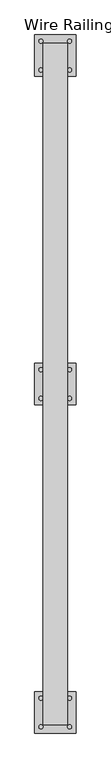
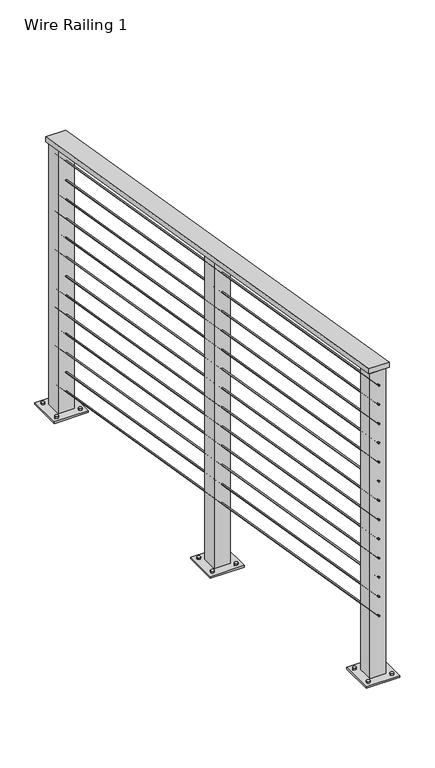
"""IFC4 building model written with IfcOpenShell, lengths in millimetres: railing geometry, Wire Railing 1."""

from ifc_helpers import new_model, si_unit, point, frame, frame_2d, origin, place, context, project, spatial, polyline, circle_curve, ellipse_curve, trimmed, segment, composite_curve, outline, extrude, faceted_brep, source, transform, mapped, element, save
from ifc_brep_helpers import plane_surface, cylinder_surface, advanced_brep


def wire_railing_1_6491a036(model_context):
    return source(origin(), model_context, "Body", "SolidModel", [
        faceted_brep([(24259.156657, 27805.7156612, 268903.5837578), (24335.356657, 27805.7156612, 268903.5837578), (24335.356657, 27805.7156612, 268884.2662422), (24259.156657, 27805.7156612, 268884.2662422), (24259.156657, 25703.8656612, 269257.0623022), (24259.156657, 25703.8656612, 269237.7447867), (24335.356657, 25703.8656612, 269237.7447867), (24335.356657, 25703.8656612, 269257.0623022)], [[[0, 1, 2, 3]], [[4, 5, 6, 7]], [[1, 0, 4, 7]], [[2, 1, 7, 6]], [[3, 2, 6, 5]], [[0, 3, 5, 4]]]),
        advanced_brep(
        [(24299.637907, 27805.7156612, 268824.8353106), (24294.875407, 27805.7156612, 268824.8353106), (24299.637907, 25703.8656612, 269178.3138551), (24294.875407, 25703.8656612, 269178.3138551)],
        [
            (0, 1, ellipse_curve(frame((24297.256657, 27805.7156612, 268824.8353106), z_axis=(0.0, 1.0, 0.0), x_axis=(0.0, 0.0, -1.0)), 2.4146894, 2.38125)),
            (1, 0, ellipse_curve(frame((24297.256657, 27805.7156612, 268824.8353106), z_axis=(0.0, 1.0, 0.0), x_axis=(0.0, 0.0, -1.0)), 2.4146894, 2.38125)),
            (2, 3, ellipse_curve(frame((24297.256657, 25703.8656612, 269178.3138551), z_axis=(0.0, -1.0, 0.0), x_axis=(0.0, 0.0, -1.0)), 2.4146894, 2.38125)),
            (3, 2, ellipse_curve(frame((24297.256657, 25703.8656612, 269178.3138551), z_axis=(0.0, -1.0, 0.0), x_axis=(0.0, 0.0, -1.0)), 2.4146894, 2.38125)),
            (0, 2),
            (3, 1),
        ],
        [
            plane_surface(frame((24297.256657, 27805.7156612, 268827.25), z_axis=(0.0, 1.0, 0.0), x_axis=(0.0, 0.0, -1.0))),
            plane_surface(frame((24297.256657, 25703.8656612, 269180.7285445), z_axis=(0.0, -1.0, 0.0), x_axis=(0.0, 0.0, -1.0))),
            cylinder_surface(frame((24297.256657, 27805.3207404, 268824.9017264), z_axis=(0.0, 0.9861516608454989, -0.1658460183774826), x_axis=(-1.0, 0.0, 0.0)), 2.38125),
        ],
        [
            (0, [[1, 2]]),
            (1, [[3, 4]]),
            (2, [[-1, 5, -4, 6]]),
            (2, [[-2, -6, -3, -5]]),
        ],
    ),
        advanced_brep(
        [(24299.637907, 27805.7156612, 268748.6353106), (24294.875407, 27805.7156612, 268748.6353106), (24299.637907, 25703.8656612, 269102.1138551), (24294.875407, 25703.8656612, 269102.1138551)],
        [
            (0, 1, ellipse_curve(frame((24297.256657, 27805.7156612, 268748.6353106), z_axis=(0.0, 1.0, 0.0), x_axis=(0.0, 0.0, -1.0)), 2.4146894, 2.38125)),
            (1, 0, ellipse_curve(frame((24297.256657, 27805.7156612, 268748.6353106), z_axis=(0.0, 1.0, 0.0), x_axis=(0.0, 0.0, -1.0)), 2.4146894, 2.38125)),
            (2, 3, ellipse_curve(frame((24297.256657, 25703.8656612, 269102.1138551), z_axis=(0.0, -1.0, 0.0), x_axis=(0.0, 0.0, -1.0)), 2.4146894, 2.38125)),
            (3, 2, ellipse_curve(frame((24297.256657, 25703.8656612, 269102.1138551), z_axis=(0.0, -1.0, 0.0), x_axis=(0.0, 0.0, -1.0)), 2.4146894, 2.38125)),
            (0, 2),
            (3, 1),
        ],
        [
            plane_surface(frame((24297.256657, 27805.7156612, 268751.05), z_axis=(0.0, 1.0, 0.0), x_axis=(0.0, 0.0, -1.0))),
            plane_surface(frame((24297.256657, 25703.8656612, 269104.5285445), z_axis=(0.0, -1.0, 0.0), x_axis=(0.0, 0.0, -1.0))),
            cylinder_surface(frame((24297.256657, 27805.3207404, 268748.7017264), z_axis=(0.0, 0.9861516608454989, -0.1658460183774826), x_axis=(-1.0, 0.0, 0.0)), 2.38125),
        ],
        [
            (0, [[1, 2]]),
            (1, [[3, 4]]),
            (2, [[-1, 5, -4, 6]]),
            (2, [[-2, -6, -3, -5]]),
        ],
    ),
        advanced_brep(
        [(24299.637907, 27805.7156612, 268672.4353106), (24294.875407, 27805.7156612, 268672.4353106), (24299.637907, 25703.8656612, 269025.9138551), (24294.875407, 25703.8656612, 269025.9138551)],
        [
            (0, 1, ellipse_curve(frame((24297.256657, 27805.7156612, 268672.4353106), z_axis=(0.0, 1.0, 0.0), x_axis=(0.0, 0.0, -1.0)), 2.4146894, 2.38125)),
            (1, 0, ellipse_curve(frame((24297.256657, 27805.7156612, 268672.4353106), z_axis=(0.0, 1.0, 0.0), x_axis=(0.0, 0.0, -1.0)), 2.4146894, 2.38125)),
            (2, 3, ellipse_curve(frame((24297.256657, 25703.8656612, 269025.9138551), z_axis=(0.0, -1.0, 0.0), x_axis=(0.0, 0.0, -1.0)), 2.4146894, 2.38125)),
            (3, 2, ellipse_curve(frame((24297.256657, 25703.8656612, 269025.9138551), z_axis=(0.0, -1.0, 0.0), x_axis=(0.0, 0.0, -1.0)), 2.4146894, 2.38125)),
            (0, 2),
            (3, 1),
        ],
        [
            plane_surface(frame((24297.256657, 27805.7156612, 268674.85), z_axis=(0.0, 1.0, 0.0), x_axis=(0.0, 0.0, -1.0))),
            plane_surface(frame((24297.256657, 25703.8656612, 269028.3285445), z_axis=(0.0, -1.0, 0.0), x_axis=(0.0, 0.0, -1.0))),
            cylinder_surface(frame((24297.256657, 27805.3207404, 268672.5017264), z_axis=(0.0, 0.9861516608454989, -0.1658460183774826), x_axis=(-1.0, 0.0, 0.0)), 2.38125),
        ],
        [
            (0, [[1, 2]]),
            (1, [[3, 4]]),
            (2, [[-1, 5, -4, 6]]),
            (2, [[-2, -6, -3, -5]]),
        ],
    ),
        advanced_brep(
        [(24299.637907, 27805.7156612, 268596.2353106), (24294.875407, 27805.7156612, 268596.2353106), (24299.637907, 25703.8656612, 268949.7138551), (24294.875407, 25703.8656612, 268949.7138551)],
        [
            (0, 1, ellipse_curve(frame((24297.256657, 27805.7156612, 268596.2353106), z_axis=(0.0, 1.0, 0.0), x_axis=(0.0, 0.0, -1.0)), 2.4146894, 2.38125)),
            (1, 0, ellipse_curve(frame((24297.256657, 27805.7156612, 268596.2353106), z_axis=(0.0, 1.0, 0.0), x_axis=(0.0, 0.0, -1.0)), 2.4146894, 2.38125)),
            (2, 3, ellipse_curve(frame((24297.256657, 25703.8656612, 268949.7138551), z_axis=(0.0, -1.0, 0.0), x_axis=(0.0, 0.0, -1.0)), 2.4146894, 2.38125)),
            (3, 2, ellipse_curve(frame((24297.256657, 25703.8656612, 268949.7138551), z_axis=(0.0, -1.0, 0.0), x_axis=(0.0, 0.0, -1.0)), 2.4146894, 2.38125)),
            (0, 2),
            (3, 1),
        ],
        [
            plane_surface(frame((24297.256657, 27805.7156612, 268598.65), z_axis=(0.0, 1.0, 0.0), x_axis=(0.0, 0.0, -1.0))),
            plane_surface(frame((24297.256657, 25703.8656612, 268952.1285445), z_axis=(0.0, -1.0, 0.0), x_axis=(0.0, 0.0, -1.0))),
            cylinder_surface(frame((24297.256657, 27805.3207404, 268596.3017264), z_axis=(0.0, 0.9861516608454989, -0.1658460183774826), x_axis=(-1.0, 0.0, 0.0)), 2.38125),
        ],
        [
            (0, [[1, 2]]),
            (1, [[3, 4]]),
            (2, [[-1, 5, -4, 6]]),
            (2, [[-2, -6, -3, -5]]),
        ],
    ),
        advanced_brep(
        [(24299.637907, 27805.7156612, 268520.0353106), (24294.875407, 27805.7156612, 268520.0353106), (24299.637907, 25703.8656612, 268873.5138551), (24294.875407, 25703.8656612, 268873.5138551)],
        [
            (0, 1, ellipse_curve(frame((24297.256657, 27805.7156612, 268520.0353106), z_axis=(0.0, 1.0, 0.0), x_axis=(0.0, 0.0, -1.0)), 2.4146894, 2.38125)),
            (1, 0, ellipse_curve(frame((24297.256657, 27805.7156612, 268520.0353106), z_axis=(0.0, 1.0, 0.0), x_axis=(0.0, 0.0, -1.0)), 2.4146894, 2.38125)),
            (2, 3, ellipse_curve(frame((24297.256657, 25703.8656612, 268873.5138551), z_axis=(0.0, -1.0, 0.0), x_axis=(0.0, 0.0, -1.0)), 2.4146894, 2.38125)),
            (3, 2, ellipse_curve(frame((24297.256657, 25703.8656612, 268873.5138551), z_axis=(0.0, -1.0, 0.0), x_axis=(0.0, 0.0, -1.0)), 2.4146894, 2.38125)),
            (0, 2),
            (3, 1),
        ],
        [
            plane_surface(frame((24297.256657, 27805.7156612, 268522.45), z_axis=(0.0, 1.0, 0.0), x_axis=(0.0, 0.0, -1.0))),
            plane_surface(frame((24297.256657, 25703.8656612, 268875.9285445), z_axis=(0.0, -1.0, 0.0), x_axis=(0.0, 0.0, -1.0))),
            cylinder_surface(frame((24297.256657, 27805.3207404, 268520.1017264), z_axis=(0.0, 0.9861516608454989, -0.1658460183774826), x_axis=(-1.0, 0.0, 0.0)), 2.38125),
        ],
        [
            (0, [[1, 2]]),
            (1, [[3, 4]]),
            (2, [[-1, 5, -4, 6]]),
            (2, [[-2, -6, -3, -5]]),
        ],
    ),
        advanced_brep(
        [(24299.637907, 27805.7156612, 268443.8353106), (24294.875407, 27805.7156612, 268443.8353106), (24299.637907, 25703.8656612, 268797.3138551), (24294.875407, 25703.8656612, 268797.3138551)],
        [
            (0, 1, ellipse_curve(frame((24297.256657, 27805.7156612, 268443.8353106), z_axis=(0.0, 1.0, 0.0), x_axis=(0.0, 0.0, -1.0)), 2.4146894, 2.38125)),
            (1, 0, ellipse_curve(frame((24297.256657, 27805.7156612, 268443.8353106), z_axis=(0.0, 1.0, 0.0), x_axis=(0.0, 0.0, -1.0)), 2.4146894, 2.38125)),
            (2, 3, ellipse_curve(frame((24297.256657, 25703.8656612, 268797.3138551), z_axis=(0.0, -1.0, 0.0), x_axis=(0.0, 0.0, -1.0)), 2.4146894, 2.38125)),
            (3, 2, ellipse_curve(frame((24297.256657, 25703.8656612, 268797.3138551), z_axis=(0.0, -1.0, 0.0), x_axis=(0.0, 0.0, -1.0)), 2.4146894, 2.38125)),
            (0, 2),
            (3, 1),
        ],
        [
            plane_surface(frame((24297.256657, 27805.7156612, 268446.25), z_axis=(0.0, 1.0, 0.0), x_axis=(0.0, 0.0, -1.0))),
            plane_surface(frame((24297.256657, 25703.8656612, 268799.7285445), z_axis=(0.0, -1.0, 0.0), x_axis=(0.0, 0.0, -1.0))),
            cylinder_surface(frame((24297.256657, 27805.3207404, 268443.9017264), z_axis=(0.0, 0.9861516608454989, -0.1658460183774826), x_axis=(-1.0, 0.0, 0.0)), 2.38125),
        ],
        [
            (0, [[1, 2]]),
            (1, [[3, 4]]),
            (2, [[-1, 5, -4, 6]]),
            (2, [[-2, -6, -3, -5]]),
        ],
    ),
        advanced_brep(
        [(24299.637907, 27805.7156612, 268367.6353106), (24294.875407, 27805.7156612, 268367.6353106), (24299.637907, 25703.8656612, 268721.1138551), (24294.875407, 25703.8656612, 268721.1138551)],
        [
            (0, 1, ellipse_curve(frame((24297.256657, 27805.7156612, 268367.6353106), z_axis=(0.0, 1.0, 0.0), x_axis=(0.0, 0.0, -1.0)), 2.4146894, 2.38125)),
            (1, 0, ellipse_curve(frame((24297.256657, 27805.7156612, 268367.6353106), z_axis=(0.0, 1.0, 0.0), x_axis=(0.0, 0.0, -1.0)), 2.4146894, 2.38125)),
            (2, 3, ellipse_curve(frame((24297.256657, 25703.8656612, 268721.1138551), z_axis=(0.0, -1.0, 0.0), x_axis=(0.0, 0.0, -1.0)), 2.4146894, 2.38125)),
            (3, 2, ellipse_curve(frame((24297.256657, 25703.8656612, 268721.1138551), z_axis=(0.0, -1.0, 0.0), x_axis=(0.0, 0.0, -1.0)), 2.4146894, 2.38125)),
            (0, 2),
            (3, 1),
        ],
        [
            plane_surface(frame((24297.256657, 27805.7156612, 268370.05), z_axis=(0.0, 1.0, 0.0), x_axis=(0.0, 0.0, -1.0))),
            plane_surface(frame((24297.256657, 25703.8656612, 268723.5285445), z_axis=(0.0, -1.0, 0.0), x_axis=(0.0, 0.0, -1.0))),
            cylinder_surface(frame((24297.256657, 27805.3207404, 268367.7017264), z_axis=(0.0, 0.9861516608454989, -0.1658460183774826), x_axis=(-1.0, 0.0, 0.0)), 2.38125),
        ],
        [
            (0, [[1, 2]]),
            (1, [[3, 4]]),
            (2, [[-1, 5, -4, 6]]),
            (2, [[-2, -6, -3, -5]]),
        ],
    ),
        advanced_brep(
        [(24299.637907, 27805.7156612, 268291.4353106), (24294.875407, 27805.7156612, 268291.4353106), (24299.637907, 25703.8656612, 268644.9138551), (24294.875407, 25703.8656612, 268644.9138551)],
        [
            (0, 1, ellipse_curve(frame((24297.256657, 27805.7156612, 268291.4353106), z_axis=(0.0, 1.0, 0.0), x_axis=(0.0, 0.0, -1.0)), 2.4146894, 2.38125)),
            (1, 0, ellipse_curve(frame((24297.256657, 27805.7156612, 268291.4353106), z_axis=(0.0, 1.0, 0.0), x_axis=(0.0, 0.0, -1.0)), 2.4146894, 2.38125)),
            (2, 3, ellipse_curve(frame((24297.256657, 25703.8656612, 268644.9138551), z_axis=(0.0, -1.0, 0.0), x_axis=(0.0, 0.0, -1.0)), 2.4146894, 2.38125)),
            (3, 2, ellipse_curve(frame((24297.256657, 25703.8656612, 268644.9138551), z_axis=(0.0, -1.0, 0.0), x_axis=(0.0, 0.0, -1.0)), 2.4146894, 2.38125)),
            (0, 2),
            (3, 1),
        ],
        [
            plane_surface(frame((24297.256657, 27805.7156612, 268293.85), z_axis=(0.0, 1.0, 0.0), x_axis=(0.0, 0.0, -1.0))),
            plane_surface(frame((24297.256657, 25703.8656612, 268647.3285445), z_axis=(0.0, -1.0, 0.0), x_axis=(0.0, 0.0, -1.0))),
            cylinder_surface(frame((24297.256657, 27805.3207404, 268291.5017264), z_axis=(0.0, 0.9861516608454989, -0.1658460183774826), x_axis=(-1.0, 0.0, 0.0)), 2.38125),
        ],
        [
            (0, [[1, 2]]),
            (1, [[3, 4]]),
            (2, [[-1, 5, -4, 6]]),
            (2, [[-2, -6, -3, -5]]),
        ],
    ),
        advanced_brep(
        [(24299.637907, 27805.7156612, 268215.2353106), (24294.875407, 27805.7156612, 268215.2353106), (24299.637907, 25703.8656612, 268568.7138551), (24294.875407, 25703.8656612, 268568.7138551)],
        [
            (0, 1, ellipse_curve(frame((24297.256657, 27805.7156612, 268215.2353106), z_axis=(0.0, 1.0, 0.0), x_axis=(0.0, 0.0, -1.0)), 2.4146894, 2.38125)),
            (1, 0, ellipse_curve(frame((24297.256657, 27805.7156612, 268215.2353106), z_axis=(0.0, 1.0, 0.0), x_axis=(0.0, 0.0, -1.0)), 2.4146894, 2.38125)),
            (2, 3, ellipse_curve(frame((24297.256657, 25703.8656612, 268568.7138551), z_axis=(0.0, -1.0, 0.0), x_axis=(0.0, 0.0, -1.0)), 2.4146894, 2.38125)),
            (3, 2, ellipse_curve(frame((24297.256657, 25703.8656612, 268568.7138551), z_axis=(0.0, -1.0, 0.0), x_axis=(0.0, 0.0, -1.0)), 2.4146894, 2.38125)),
            (0, 2),
            (3, 1),
        ],
        [
            plane_surface(frame((24297.256657, 27805.7156612, 268217.65), z_axis=(0.0, 1.0, 0.0), x_axis=(0.0, 0.0, -1.0))),
            plane_surface(frame((24297.256657, 25703.8656612, 268571.1285445), z_axis=(0.0, -1.0, 0.0), x_axis=(0.0, 0.0, -1.0))),
            cylinder_surface(frame((24297.256657, 27805.3207404, 268215.3017264), z_axis=(0.0, 0.9861516608454989, -0.1658460183774826), x_axis=(-1.0, 0.0, 0.0)), 2.38125),
        ],
        [
            (0, [[1, 2]]),
            (1, [[3, 4]]),
            (2, [[-1, 5, -4, 6]]),
            (2, [[-2, -6, -3, -5]]),
        ],
    ),
        advanced_brep(
        [(24299.637907, 27805.7156612, 268139.0353106), (24294.875407, 27805.7156612, 268139.0353106), (24299.637907, 25703.8656612, 268492.5138551), (24294.875407, 25703.8656612, 268492.5138551)],
        [
            (0, 1, ellipse_curve(frame((24297.256657, 27805.7156612, 268139.0353106), z_axis=(0.0, 1.0, 0.0), x_axis=(0.0, 0.0, -1.0)), 2.4146894, 2.38125)),
            (1, 0, ellipse_curve(frame((24297.256657, 27805.7156612, 268139.0353106), z_axis=(0.0, 1.0, 0.0), x_axis=(0.0, 0.0, -1.0)), 2.4146894, 2.38125)),
            (2, 3, ellipse_curve(frame((24297.256657, 25703.8656612, 268492.5138551), z_axis=(0.0, -1.0, 0.0), x_axis=(0.0, 0.0, -1.0)), 2.4146894, 2.38125)),
            (3, 2, ellipse_curve(frame((24297.256657, 25703.8656612, 268492.5138551), z_axis=(0.0, -1.0, 0.0), x_axis=(0.0, 0.0, -1.0)), 2.4146894, 2.38125)),
            (0, 2),
            (3, 1),
        ],
        [
            plane_surface(frame((24297.256657, 27805.7156612, 268141.45), z_axis=(0.0, 1.0, 0.0), x_axis=(0.0, 0.0, -1.0))),
            plane_surface(frame((24297.256657, 25703.8656612, 268494.9285445), z_axis=(0.0, -1.0, 0.0), x_axis=(0.0, 0.0, -1.0))),
            cylinder_surface(frame((24297.256657, 27805.3207404, 268139.1017264), z_axis=(0.0, 0.9861516608454989, -0.1658460183774826), x_axis=(-1.0, 0.0, 0.0)), 2.38125),
        ],
        [
            (0, [[1, 2]]),
            (1, [[3, 4]]),
            (2, [[-1, 5, -4, 6]]),
            (2, [[-2, -6, -3, -5]]),
        ],
    ),
        advanced_brep(
        [(24299.637907, 27805.7156612, 268062.8353106), (24294.875407, 27805.7156612, 268062.8353106), (24299.637907, 25703.8656612, 268416.3138551), (24294.875407, 25703.8656612, 268416.3138551)],
        [
            (0, 1, ellipse_curve(frame((24297.256657, 27805.7156612, 268062.8353106), z_axis=(0.0, 1.0, 0.0), x_axis=(0.0, 0.0, -1.0)), 2.4146894, 2.38125)),
            (1, 0, ellipse_curve(frame((24297.256657, 27805.7156612, 268062.8353106), z_axis=(0.0, 1.0, 0.0), x_axis=(0.0, 0.0, -1.0)), 2.4146894, 2.38125)),
            (2, 3, ellipse_curve(frame((24297.256657, 25703.8656612, 268416.3138551), z_axis=(0.0, -1.0, 0.0), x_axis=(0.0, 0.0, -1.0)), 2.4146894, 2.38125)),
            (3, 2, ellipse_curve(frame((24297.256657, 25703.8656612, 268416.3138551), z_axis=(0.0, -1.0, 0.0), x_axis=(0.0, 0.0, -1.0)), 2.4146894, 2.38125)),
            (0, 2),
            (3, 1),
        ],
        [
            plane_surface(frame((24297.256657, 27805.7156612, 268065.25), z_axis=(0.0, 1.0, 0.0), x_axis=(0.0, 0.0, -1.0))),
            plane_surface(frame((24297.256657, 25703.8656612, 268418.7285445), z_axis=(0.0, -1.0, 0.0), x_axis=(0.0, 0.0, -1.0))),
            cylinder_surface(frame((24297.256657, 27805.3207404, 268062.9017264), z_axis=(0.0, 0.9861516608454989, -0.1658460183774826), x_axis=(-1.0, 0.0, 0.0)), 2.38125),
        ],
        [
            (0, [[1, 2]]),
            (1, [[3, 4]]),
            (2, [[-1, 5, -4, 6]]),
            (2, [[-2, -6, -3, -5]]),
        ],
    ),
        advanced_brep(
        [(24299.637907, 27805.7156612, 267986.6353106), (24294.875407, 27805.7156612, 267986.6353106), (24299.637907, 25703.8656612, 268340.1138551), (24294.875407, 25703.8656612, 268340.1138551)],
        [
            (0, 1, ellipse_curve(frame((24297.256657, 27805.7156612, 267986.6353106), z_axis=(0.0, 1.0, 0.0), x_axis=(0.0, 0.0, -1.0)), 2.4146894, 2.38125)),
            (1, 0, ellipse_curve(frame((24297.256657, 27805.7156612, 267986.6353106), z_axis=(0.0, 1.0, 0.0), x_axis=(0.0, 0.0, -1.0)), 2.4146894, 2.38125)),
            (2, 3, ellipse_curve(frame((24297.256657, 25703.8656612, 268340.1138551), z_axis=(0.0, -1.0, 0.0), x_axis=(0.0, 0.0, -1.0)), 2.4146894, 2.38125)),
            (3, 2, ellipse_curve(frame((24297.256657, 25703.8656612, 268340.1138551), z_axis=(0.0, -1.0, 0.0), x_axis=(0.0, 0.0, -1.0)), 2.4146894, 2.38125)),
            (0, 2),
            (3, 1),
        ],
        [
            plane_surface(frame((24297.256657, 27805.7156612, 267989.05), z_axis=(0.0, 1.0, 0.0), x_axis=(0.0, 0.0, -1.0))),
            plane_surface(frame((24297.256657, 25703.8656612, 268342.5285445), z_axis=(0.0, -1.0, 0.0), x_axis=(0.0, 0.0, -1.0))),
            cylinder_surface(frame((24297.256657, 27805.3207404, 267986.7017264), z_axis=(0.0, 0.9861516608454989, -0.1658460183774826), x_axis=(-1.0, 0.0, 0.0)), 2.38125),
        ],
        [
            (0, [[1, 2]]),
            (1, [[3, 4]]),
            (2, [[-1, 5, -4, 6]]),
            (2, [[-2, -6, -3, -5]]),
        ],
    ),
        advanced_brep(
        [(24299.637907, 27805.7156612, 267910.4353106), (24294.875407, 27805.7156612, 267910.4353106), (24299.637907, 25703.8656612, 268263.9138551), (24294.875407, 25703.8656612, 268263.9138551)],
        [
            (0, 1, ellipse_curve(frame((24297.256657, 27805.7156612, 267910.4353106), z_axis=(0.0, 1.0, 0.0), x_axis=(0.0, 0.0, -1.0)), 2.4146894, 2.38125)),
            (1, 0, ellipse_curve(frame((24297.256657, 27805.7156612, 267910.4353106), z_axis=(0.0, 1.0, 0.0), x_axis=(0.0, 0.0, -1.0)), 2.4146894, 2.38125)),
            (2, 3, ellipse_curve(frame((24297.256657, 25703.8656612, 268263.9138551), z_axis=(0.0, -1.0, 0.0), x_axis=(0.0, 0.0, -1.0)), 2.4146894, 2.38125)),
            (3, 2, ellipse_curve(frame((24297.256657, 25703.8656612, 268263.9138551), z_axis=(0.0, -1.0, 0.0), x_axis=(0.0, 0.0, -1.0)), 2.4146894, 2.38125)),
            (0, 2),
            (3, 1),
        ],
        [
            plane_surface(frame((24297.256657, 27805.7156612, 267912.85), z_axis=(0.0, 1.0, 0.0), x_axis=(0.0, 0.0, -1.0))),
            plane_surface(frame((24297.256657, 25703.8656612, 268266.3285445), z_axis=(0.0, -1.0, 0.0), x_axis=(0.0, 0.0, -1.0))),
            cylinder_surface(frame((24297.256657, 27805.3207404, 267910.5017264), z_axis=(0.0, 0.9861516608454989, -0.1658460183774826), x_axis=(-1.0, 0.0, 0.0)), 2.38125),
        ],
        [
            (0, [[1, 2]]),
            (1, [[3, 4]]),
            (2, [[-1, 5, -4, 6]]),
            (2, [[-2, -6, -3, -5]]),
        ],
    ),
        extrude(outline(polyline([(24327.419157, 26784.9531612), (24327.419157, 26724.6281612), (24267.094157, 26724.6281612), (24267.094157, 26784.9531612), (24327.419157, 26784.9531612)]), holes=[polyline([(24321.069157, 26778.6031612), (24273.444157, 26778.6031612), (24273.444157, 26730.9781612), (24321.069157, 26730.9781612), (24321.069157, 26778.6031612)])]), frame((0.0, 0.0, 267836.65), z_axis=(0.0, 0.0, 1.0), x_axis=(1.0, 0.0, 0.0)), (0.0, 0.0, 1.0), 1224.3555145),
        extrude(outline(composite_curve([segment(trimmed(circle_curve(frame_2d((24252.806657, 26799.2406612)), 6.35), [point((24246.456657, 26799.2406612))], [point((24259.156657, 26799.2406612))], False, "CARTESIAN"), True, "CONTINUOUS"), segment(trimmed(circle_curve(frame_2d((24252.806657, 26799.2406612)), 6.35), [point((24259.156657, 26799.2406612))], [point((24246.456657, 26799.2406612))], False, "CARTESIAN"), True, "CONTINUOUS")], self_intersect=False)), frame((0.0, 0.0, 267836.65), z_axis=(0.0, 0.0, 1.0), x_axis=(1.0, 0.0, 0.0)), (0.0, 0.0, 1.0), 12.7),
        extrude(outline(composite_curve([segment(trimmed(circle_curve(frame_2d((24341.706657, 26799.2406612)), 6.35), [point((24335.356657, 26799.2406612))], [point((24348.056657, 26799.2406612))], False, "CARTESIAN"), True, "CONTINUOUS"), segment(trimmed(circle_curve(frame_2d((24341.706657, 26799.2406612)), 6.35), [point((24348.056657, 26799.2406612))], [point((24335.356657, 26799.2406612))], False, "CARTESIAN"), True, "CONTINUOUS")], self_intersect=False)), frame((0.0, 0.0, 267836.65), z_axis=(0.0, 0.0, 1.0), x_axis=(1.0, 0.0, 0.0)), (0.0, 0.0, 1.0), 12.7),
        extrude(outline(composite_curve([segment(trimmed(circle_curve(frame_2d((24252.806657, 26710.3406612)), 6.35), [point((24246.456657, 26710.3406612))], [point((24259.156657, 26710.3406612))], False, "CARTESIAN"), True, "CONTINUOUS"), segment(trimmed(circle_curve(frame_2d((24252.806657, 26710.3406612)), 6.35), [point((24259.156657, 26710.3406612))], [point((24246.456657, 26710.3406612))], False, "CARTESIAN"), True, "CONTINUOUS")], self_intersect=False)), frame((0.0, 0.0, 267836.65), z_axis=(0.0, 0.0, 1.0), x_axis=(1.0, 0.0, 0.0)), (0.0, 0.0, 1.0), 12.7),
        extrude(outline(composite_curve([segment(trimmed(circle_curve(frame_2d((24341.706657, 26710.3406612)), 6.35), [point((24335.356657, 26710.3406612))], [point((24348.056657, 26710.3406612))], False, "CARTESIAN"), True, "CONTINUOUS"), segment(trimmed(circle_curve(frame_2d((24341.706657, 26710.3406612)), 6.35), [point((24348.056657, 26710.3406612))], [point((24335.356657, 26710.3406612))], False, "CARTESIAN"), True, "CONTINUOUS")], self_intersect=False)), frame((0.0, 0.0, 267836.65), z_axis=(0.0, 0.0, 1.0), x_axis=(1.0, 0.0, 0.0)), (0.0, 0.0, 1.0), 12.7),
        extrude(outline(polyline([(24360.756657, 26818.2906612), (24360.756657, 26691.2906612), (24233.756657, 26691.2906612), (24233.756657, 26818.2906612), (24360.756657, 26818.2906612)])), frame((0.0, 0.0, 267836.65), z_axis=(0.0, 0.0, 1.0), x_axis=(1.0, 0.0, 0.0)), (0.0, 0.0, 1.0), 6.35),
        extrude(outline(composite_curve([segment(trimmed(circle_curve(frame_2d((24252.806657, 25786.4156612)), 6.35), [point((24246.456657, 25786.4156612))], [point((24259.156657, 25786.4156612))], False, "CARTESIAN"), True, "CONTINUOUS"), segment(trimmed(circle_curve(frame_2d((24252.806657, 25786.4156612)), 6.35), [point((24259.156657, 25786.4156612))], [point((24246.456657, 25786.4156612))], False, "CARTESIAN"), True, "CONTINUOUS")], self_intersect=False)), frame((0.0, 0.0, 268013.65625), z_axis=(0.0, 0.0, 1.0), x_axis=(1.0, 0.0, 0.0)), (0.0, 0.0, 1.0), 12.7),
        extrude(outline(composite_curve([segment(trimmed(circle_curve(frame_2d((24341.706657, 25786.4156612)), 6.35), [point((24335.356657, 25786.4156612))], [point((24348.056657, 25786.4156612))], False, "CARTESIAN"), True, "CONTINUOUS"), segment(trimmed(circle_curve(frame_2d((24341.706657, 25786.4156612)), 6.35), [point((24348.056657, 25786.4156612))], [point((24335.356657, 25786.4156612))], False, "CARTESIAN"), True, "CONTINUOUS")], self_intersect=False)), frame((0.0, 0.0, 268013.65625), z_axis=(0.0, 0.0, 1.0), x_axis=(1.0, 0.0, 0.0)), (0.0, 0.0, 1.0), 12.7),
        extrude(outline(composite_curve([segment(trimmed(circle_curve(frame_2d((24252.806657, 25697.5156612)), 6.35), [point((24246.456657, 25697.5156612))], [point((24259.156657, 25697.5156612))], False, "CARTESIAN"), True, "CONTINUOUS"), segment(trimmed(circle_curve(frame_2d((24252.806657, 25697.5156612)), 6.35), [point((24259.156657, 25697.5156612))], [point((24246.456657, 25697.5156612))], False, "CARTESIAN"), True, "CONTINUOUS")], self_intersect=False)), frame((0.0, 0.0, 268013.65625), z_axis=(0.0, 0.0, 1.0), x_axis=(1.0, 0.0, 0.0)), (0.0, 0.0, 1.0), 12.7),
        extrude(outline(composite_curve([segment(trimmed(circle_curve(frame_2d((24341.706657, 25697.5156612)), 6.35), [point((24335.356657, 25697.5156612))], [point((24348.056657, 25697.5156612))], False, "CARTESIAN"), True, "CONTINUOUS"), segment(trimmed(circle_curve(frame_2d((24341.706657, 25697.5156612)), 6.35), [point((24348.056657, 25697.5156612))], [point((24335.356657, 25697.5156612))], False, "CARTESIAN"), True, "CONTINUOUS")], self_intersect=False)), frame((0.0, 0.0, 268013.65625), z_axis=(0.0, 0.0, 1.0), x_axis=(1.0, 0.0, 0.0)), (0.0, 0.0, 1.0), 12.7),
        extrude(outline(polyline([(24360.756657, 25805.4656612), (24360.756657, 25678.4656612), (24233.756657, 25678.4656612), (24233.756657, 25805.4656612), (24360.756657, 25805.4656612)])), frame((0.0, 0.0, 268013.65625), z_axis=(0.0, 0.0, 1.0), x_axis=(1.0, 0.0, 0.0)), (0.0, 0.0, 1.0), 6.35),
        extrude(outline(polyline([(24327.419157, 25772.1281612), (24327.419157, 25711.8031612), (24267.094157, 25711.8031612), (24267.094157, 25772.1281612), (24327.419157, 25772.1281612)]), holes=[polyline([(24321.069157, 25765.7781612), (24273.444157, 25765.7781612), (24273.444157, 25718.1531612), (24321.069157, 25718.1531612), (24321.069157, 25765.7781612)])]), frame((0.0, 0.0, 268013.65625), z_axis=(0.0, 0.0, 1.0), x_axis=(1.0, 0.0, 0.0)), (0.0, 0.0, 1.0), 1217.6810707),
        extrude(outline(composite_curve([segment(trimmed(circle_curve(frame_2d((24252.806657, 27812.0656612)), 6.35), [point((24246.456657, 27812.0656612))], [point((24259.156657, 27812.0656612))], False, "CARTESIAN"), True, "CONTINUOUS"), segment(trimmed(circle_curve(frame_2d((24252.806657, 27812.0656612)), 6.35), [point((24259.156657, 27812.0656612))], [point((24246.456657, 27812.0656612))], False, "CARTESIAN"), True, "CONTINUOUS")], self_intersect=False)), frame((0.0, 0.0, 267836.65), z_axis=(0.0, 0.0, 1.0), x_axis=(1.0, 0.0, 0.0)), (0.0, 0.0, 1.0), 12.7),
        extrude(outline(composite_curve([segment(trimmed(circle_curve(frame_2d((24341.706657, 27812.0656612)), 6.35), [point((24335.356657, 27812.0656612))], [point((24348.056657, 27812.0656612))], False, "CARTESIAN"), True, "CONTINUOUS"), segment(trimmed(circle_curve(frame_2d((24341.706657, 27812.0656612)), 6.35), [point((24348.056657, 27812.0656612))], [point((24335.356657, 27812.0656612))], False, "CARTESIAN"), True, "CONTINUOUS")], self_intersect=False)), frame((0.0, 0.0, 267836.65), z_axis=(0.0, 0.0, 1.0), x_axis=(1.0, 0.0, 0.0)), (0.0, 0.0, 1.0), 12.7),
        extrude(outline(composite_curve([segment(trimmed(circle_curve(frame_2d((24252.806657, 27723.1656612)), 6.35), [point((24246.456657, 27723.1656612))], [point((24259.156657, 27723.1656612))], False, "CARTESIAN"), True, "CONTINUOUS"), segment(trimmed(circle_curve(frame_2d((24252.806657, 27723.1656612)), 6.35), [point((24259.156657, 27723.1656612))], [point((24246.456657, 27723.1656612))], False, "CARTESIAN"), True, "CONTINUOUS")], self_intersect=False)), frame((0.0, 0.0, 267836.65), z_axis=(0.0, 0.0, 1.0), x_axis=(1.0, 0.0, 0.0)), (0.0, 0.0, 1.0), 12.7),
        extrude(outline(composite_curve([segment(trimmed(circle_curve(frame_2d((24341.706657, 27723.1656612)), 6.35), [point((24335.356657, 27723.1656612))], [point((24348.056657, 27723.1656612))], False, "CARTESIAN"), True, "CONTINUOUS"), segment(trimmed(circle_curve(frame_2d((24341.706657, 27723.1656612)), 6.35), [point((24348.056657, 27723.1656612))], [point((24335.356657, 27723.1656612))], False, "CARTESIAN"), True, "CONTINUOUS")], self_intersect=False)), frame((0.0, 0.0, 267836.65), z_axis=(0.0, 0.0, 1.0), x_axis=(1.0, 0.0, 0.0)), (0.0, 0.0, 1.0), 12.7),
        extrude(outline(polyline([(24360.756657, 27831.1156612), (24360.756657, 27704.1156612), (24233.756657, 27704.1156612), (24233.756657, 27831.1156612), (24360.756657, 27831.1156612)])), frame((0.0, 0.0, 267836.65), z_axis=(0.0, 0.0, 1.0), x_axis=(1.0, 0.0, 0.0)), (0.0, 0.0, 1.0), 6.35),
        extrude(outline(polyline([(24327.419157, 27797.7781612), (24327.419157, 27737.4531612), (24267.094157, 27737.4531612), (24267.094157, 27797.7781612), (24327.419157, 27797.7781612)]), holes=[polyline([(24321.069157, 27791.4281612), (24273.444157, 27791.4281612), (24273.444157, 27743.8031612), (24321.069157, 27743.8031612), (24321.069157, 27791.4281612)])]), frame((0.0, 0.0, 267836.65), z_axis=(0.0, 0.0, 1.0), x_axis=(1.0, 0.0, 0.0)), (0.0, 0.0, 1.0), 1054.0237083),
    ])


if __name__ == "__main__":
    model = new_model("IFC4")
    model_context = context("Model", 3, world=origin())
    ifc_project = project(units=[si_unit("LENGTHUNIT", "METRE", prefix="MILLI")], contexts=[model_context])
    site = spatial("IfcSite", under=ifc_project)
    building = spatial("IfcBuilding", under=site)
    placement = place(None, origin())
    wire_railing_1_shape = wire_railing_1_6491a036(model_context)
    element("IfcRailing", 1, ObjectType="Wire Railing 1", at=placement, inside=building, context=model_context, shape_type="MappedRepresentation", body=[
        mapped(wire_railing_1_shape, transform((0.0, 0.0, 0.0), x_axis=(1.0, 0.0, 0.0), y_axis=(0.0, 1.0, 0.0), z_axis=(0.0, 0.0, 1.0))),
    ])
    save(model, "model.ifc")

# Revit data of these elements
# Element 1 (IfcRailing, "Wire Railing 1")
#   Materials on its faces: "2 1/2\" X 2 1/2\" ALUM. SQUARE POST (38\" O.C. MAX)", "WIRE RAILING (3\" O.C.)", "ALUM. PLATE TOP RAIL"
# Materials
#   "2 1/2\" X 2 1/2\" ALUM. SQUARE POST (38\" O.C. MAX)": class "Metal", colour RGB 244 244 244, transparency 0, Manufacturer = "Kawneer", URL = "http://www.kawneer.com/kawneer/north_america/en/home.asp", Cost = 0
#   "WIRE RAILING (3\" O.C.)": class "Metal", colour RGB 244 244 244, transparency 0, Manufacturer = "Kawneer", URL = "http://www.kawneer.com/kawneer/north_america/en/home.asp", Cost = 0
#   "ALUM. PLATE TOP RAIL": class "Metal", colour RGB 244 244 244, transparency 0, Manufacturer = "Kawneer", URL = "http://www.kawneer.com/kawneer/north_america/en/home.asp", Cost = 0
